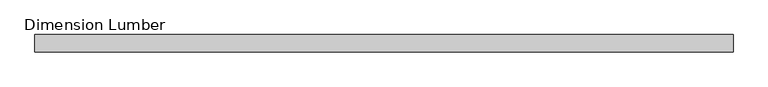
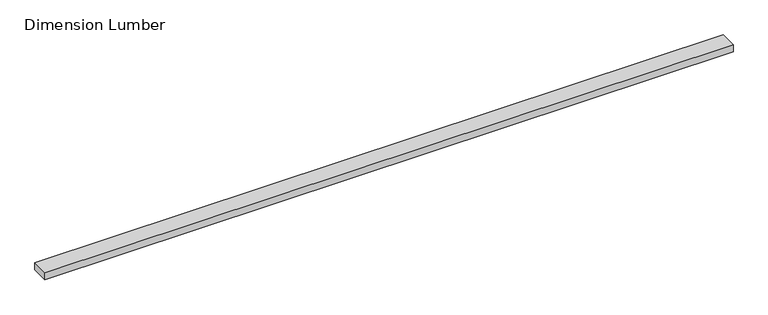
"""IFC4 building model written with IfcOpenShell, lengths in millimetres: beam geometry, Dimension Lumber : Top Supporting Lumbers."""

from ifc_helpers import new_model, si_unit, frame, origin, place, context, project, spatial, polyline, outline, extrude, source, transform, mapped, element, save


def dimension_lumber_a9f99430(model_context):
    return source(origin(), model_context, "Body", "SweptSolid", [
        extrude(outline(polyline([(1762.125, 44.45), (1762.125, -44.45), (-1778.0, -44.45), (-1778.0, 44.45), (1762.125, 44.45)])), frame((0.0, 0.0, -19.05), z_axis=(0.0, 0.0, 1.0), x_axis=(1.0, 0.0, 0.0)), (0.0, 0.0, 1.0), 38.1),
    ])


if __name__ == "__main__":
    model = new_model("IFC4")
    model_context = context("Model", 3, world=origin())
    ifc_project = project(units=[si_unit("LENGTHUNIT", "METRE", prefix="MILLI")], contexts=[model_context])
    site = spatial("IfcSite", under=ifc_project)
    building = spatial("IfcBuilding", under=site)
    placement = place(None, origin())
    dimension_lumber_shape = dimension_lumber_a9f99430(model_context)
    element("IfcBeam", 1, ObjectType="Dimension Lumber : Top Supporting Lumbers", at=placement, inside=building, context=model_context, shape_type="MappedRepresentation", body=[
        mapped(dimension_lumber_shape, transform((0.0, 0.0, 0.0), x_axis=(1.0, 0.0, 0.0), y_axis=(0.0, 1.0, 0.0), z_axis=(0.0, 0.0, 1.0))),
    ])
    save(model, "model.ifc")

# Revit data of these elements
# Type "Dimension Lumber : Top Supporting Lumbers"
#   Assembly Code = "B10"
#   A = 0.0364583 SF
#   Length [instance default] = 5' - 0"
#   b = 0' - 3 1/2"
#   d = 0' - 1 1/2"
#   Structural Material [instance default] = Softwood, Lumber
# Element 1 (IfcBeam, "Dimension Lumber : Top Supporting Lumbers")
#   Structural Material = Douglas Fir #2
#   Materials on its faces: "Douglas Fir #2"
# Materials
#   "Softwood, Lumber": class "Wood", colour RGB 223 192 134, transparency 0, Description = "Pinus Echinata", Cost = 0
#   "Douglas Fir #2": class "Wood", colour RGB 223 192 134, transparency 0, Description = "Pinus Echinata", Cost = 0
